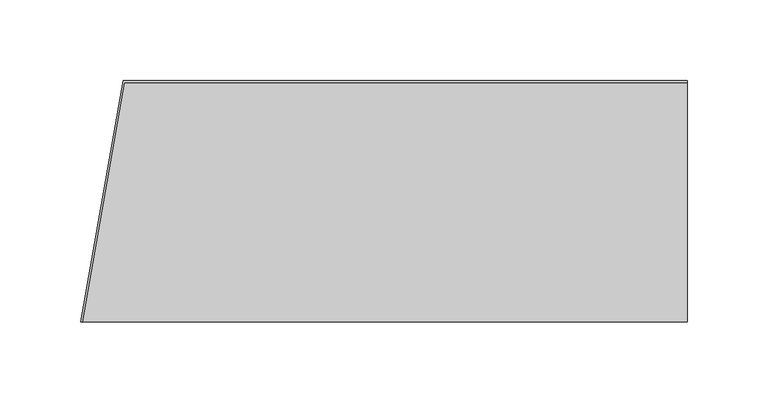
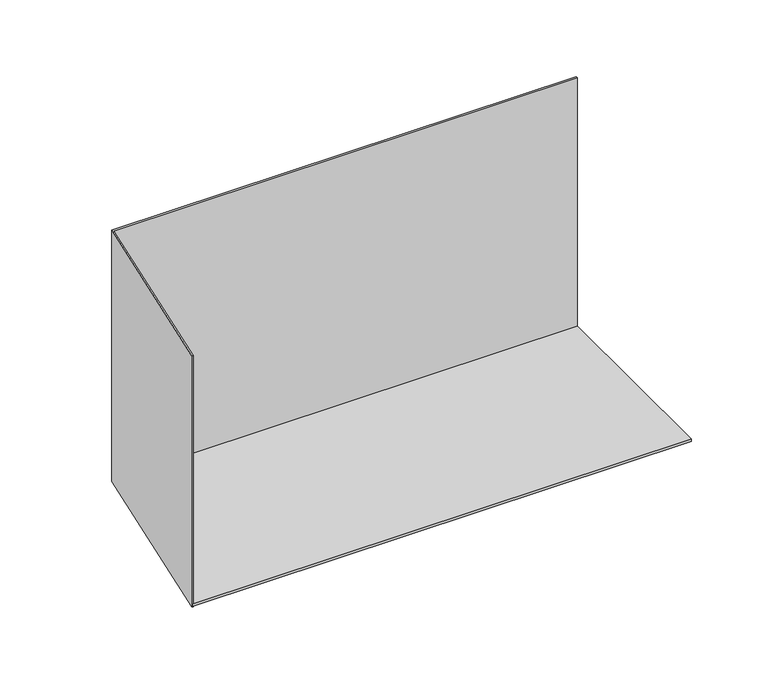
"""IFC4 building model written with IfcOpenShell, lengths in millimetres: proxy geometry, TN_ПВС 125-82_Пристенный поворотный отлив карнизного свеса : TN_ПВС 125-82_Пристенный поворотный отлив карнизного свеса."""

from ifc_helpers import new_model, si_unit, origin, place, context, project, spatial, faceted_brep, source, transform, mapped, element, save


def generic_models_81dd5289(model_context):
    return source(origin(), model_context, "Body", "Brep", [
        faceted_brep([(350.0, 0.0, 0.0), (350.0, 0.0, 200.0), (350.0, -1.3333333, 200.0), (350.0, -1.3333333, 2.0), (350.0, -150.0, 2.0), (350.0, -150.0, 0.0), (0.0, 0.0, 0.0), (0.0, 0.0, 200.0), (-26.4490471, -150.0, 200.0), (-25.4642394, -150.1736482, 200.0), (0.780324, -1.3333333, 200.0), (0.780324, -1.3333333, 2.0), (-25.4336205, -150.0, 2.0), (-25.4336205, -150.0, 0.0), (-25.4642394, -150.1736482, 0.0), (-26.4490471, -150.0, 0.0)], [[[0, 1, 2, 3, 4, 5]], [[1, 0, 6, 7]], [[2, 1, 7, 8, 9, 10]], [[3, 2, 10, 11]], [[4, 3, 11, 12]], [[5, 4, 12, 13]], [[0, 5, 13, 14, 15, 6]], [[6, 15, 8, 7]], [[9, 14, 13, 12, 11, 10]], [[9, 8, 15, 14]]]),
    ])


if __name__ == "__main__":
    model = new_model("IFC4")
    model_context = context("Model", 3, world=origin())
    ifc_project = project(units=[si_unit("LENGTHUNIT", "METRE", prefix="MILLI")], contexts=[model_context])
    site = spatial("IfcSite", under=ifc_project)
    building = spatial("IfcBuilding", under=site)
    placement = place(None, origin())
    generic_models_shape = generic_models_81dd5289(model_context)
    element("IfcBuildingElementProxy", 1, Name="TN_ПВС 125-82_Пристенный поворотный отлив карнизного свеса : TN_ПВС 125-82_Пристенный поворотный отлив карнизного свеса", ObjectType="TN_ПВС 125-82_Пристенный поворотный отлив карнизного свеса : TN_ПВС 125-82_Пристенный поворотный отлив карнизного свеса", at=placement, inside=building, context=model_context, shape_type="MappedRepresentation", body=[
        mapped(generic_models_shape, transform((0.0, 0.0, 0.0), x_axis=(1.0, 0.0, 0.0), y_axis=(0.0, 1.0, 0.0), z_axis=(0.0, 0.0, 1.0))),
    ])
    save(model, "model.ifc")

# Revit data of these elements
# Type "TN_ПВС 125-82_Пристенный поворотный отлив карнизного свеса : TN_ПВС 125-82_Пристенный поворотный отлив карнизного свеса"
#   Description = "Оформление примыкания ската кровли к вертикальной\r\nстене здания"
#   Manufacturer = "ТехноНИКОЛЬ"
#   Model = "Комплектующие к водосточным системам"
#   URL = "https://tn-vodostok.ru/catalog/pvh/"
#   ADSK_Обозначение = "ТехноНИКОЛЬ"
#   ADSK_Наименование краткое = "Пристенный отлив"
#   ADSK_Наименование = "Пристенный поворотный отлив карнизного свеса"
#   ADSK_Масса_Текст = ""
#   ADSK_Марка = ""
#   ADSK_Код изделия = ""
#   ADSK_Завод-изготовитель = "ТехноНИКОЛЬ"
#   ADSK_Единица измерения = "шт."
#   ADSK_Группирование = "Комплектующие к водосточным системам"
#   ADSK_URL страницы изделия = "https://tn-vodostok.ru/catalog/pvh/"
#   ADSK_URL документации изделия = "https://tn-vodostok.ru/upload/iblock/c42/c427963cb77eb5c3c51f0cfb870e9e52.pdf"
#   Угол поворота [instance default] = 10.00°
#   Длина дополнительная [instance default] = 152.314 mm
#   ADSK_Размер_Ширина = 350 mm
#   ADSK_Размер_Глубина = 150 mm
#   ADSK_Размер_Высота = 200 mm
#   ADSK_Количество = 1
#   ADSK_Материал = TN_Пластик_Белый_RAL9010
#   Default Elevation = 0
# Element 1 (IfcBuildingElementProxy, "TN_ПВС 125-82_Пристенный поворотный отлив карнизного свеса : TN_ПВС 125-82_Пристенный поворотный отлив карнизного свеса")
#   Materials on its faces: "TN_Пластик_Белый_RAL9010"
# Materials
#   "TN_Пластик_Белый_RAL9010": class "Типовые", colour RGB 241 236 225, transparency 0, Cost = 0
